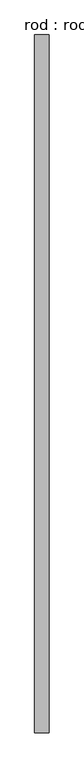
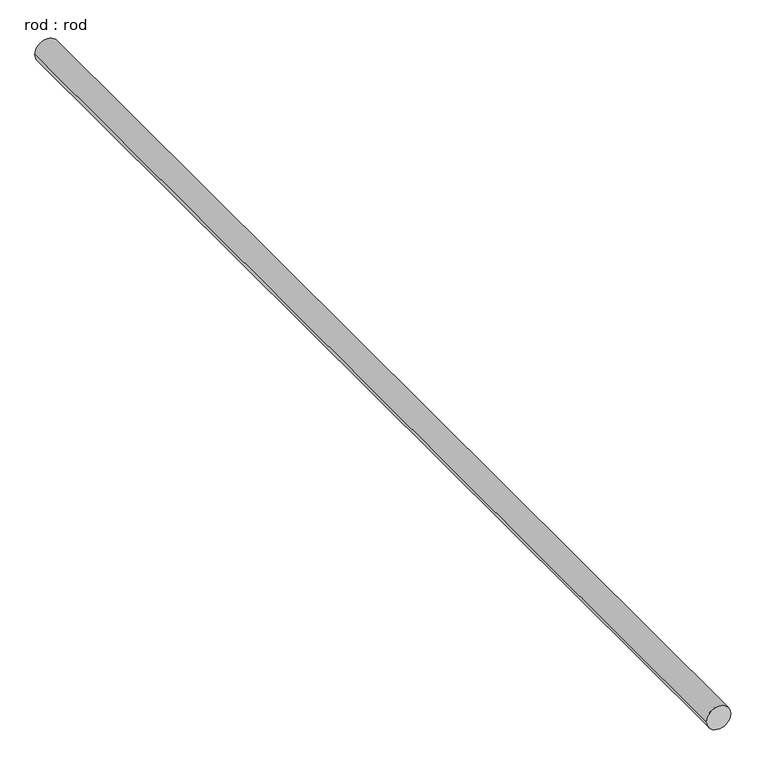
"""IFC4 building model written with IfcOpenShell, lengths in millimetres: proxy geometry, rod : rod."""

from ifc_helpers import new_model, si_unit, point, frame, frame_2d, origin, place, context, project, spatial, circle_curve, trimmed, segment, composite_curve, outline, extrude, source, transform, mapped, element, save


def rod_rod_1ffcb5c5(model_context):
    return source(origin(), model_context, "Body", "SweptSolid", [
        extrude(outline(composite_curve([segment(trimmed(circle_curve(frame_2d((0.0108462, 0.0)), 200.0), [point((0.0108462, 200.0))], [point((0.0108462, -200.0))], False, "CARTESIAN"), True, "CONTINUOUS"), segment(trimmed(circle_curve(frame_2d((0.0108462, 0.0)), 200.0), [point((0.0108462, -200.0))], [point((0.0108462, 200.0))], False, "CARTESIAN"), True, "CONTINUOUS")], self_intersect=False)), frame((0.0, -5490.604718, 0.0), z_axis=(0.0, 1.0, 0.0), x_axis=(0.0, 0.0, 1.0)), (0.0, 0.0, 1.0), 19166.6666667),
    ])


if __name__ == "__main__":
    model = new_model("IFC4")
    model_context = context("Model", 3, world=origin())
    ifc_project = project(units=[si_unit("LENGTHUNIT", "METRE", prefix="MILLI")], contexts=[model_context])
    site = spatial("IfcSite", under=ifc_project)
    building = spatial("IfcBuilding", under=site)
    placement = place(None, origin())
    rod_rod_shape = rod_rod_1ffcb5c5(model_context)
    element("IfcBuildingElementProxy", 1, Name="rod : rod", ObjectType="rod : rod", at=placement, inside=building, context=model_context, shape_type="MappedRepresentation", body=[
        mapped(rod_rod_shape, transform((0.0, 0.0, 0.0), x_axis=(1.0, 0.0, 0.0), y_axis=(0.0, 1.0, 0.0), z_axis=(0.0, 0.0, 1.0))),
    ])
    save(model, "model.ifc")

# Revit data of these elements
# Type "rod : rod"
#   Default Elevation = 0
